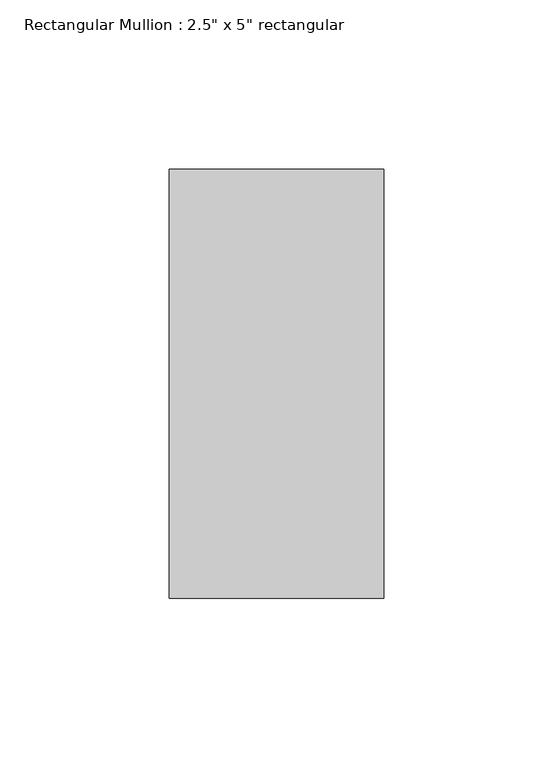
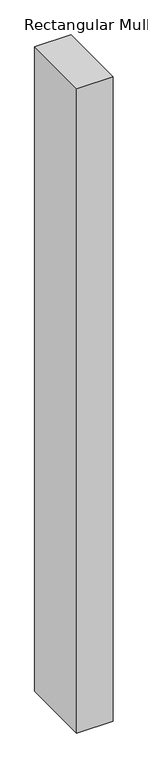
"""IFC4 building model written with IfcOpenShell, lengths in millimetres: member geometry."""

from ifc_helpers import new_model, si_unit, frame, origin, place, context, project, spatial, polyline, outline, extrude, source, transform, mapped, element, save


def member_c617b399(model_context):
    return source(origin(), model_context, "Body", "SweptSolid", [
        extrude(outline(polyline([(0.0, 63.5), (0.0, -63.5), (-63.5, -63.5), (-63.5, 63.5), (0.0, 63.5)])), frame((0.0, 0.0, -1188.8151287), z_axis=(0.0, 0.0, 1.0), x_axis=(1.0, 0.0, 0.0)), (0.0, 0.0, 1.0), 1188.8151287),
    ])


if __name__ == "__main__":
    model = new_model("IFC4")
    model_context = context("Model", 3, world=origin())
    ifc_project = project(units=[si_unit("LENGTHUNIT", "METRE", prefix="MILLI")], contexts=[model_context])
    site = spatial("IfcSite", under=ifc_project)
    building = spatial("IfcBuilding", under=site)
    placement = place(None, origin())
    member_shape = member_c617b399(model_context)
    element("IfcMember", 1, ObjectType="Rectangular Mullion : 2.5\" x 5\" rectangular", at=placement, inside=building, context=model_context, shape_type="MappedRepresentation", body=[
        mapped(member_shape, transform((0.0, 0.0, 0.0), x_axis=(1.0, 0.0, 0.0), y_axis=(0.0, 1.0, 0.0), z_axis=(0.0, 0.0, 1.0))),
    ])
    save(model, "model.ifc")

# Revit data of these elements
# Type "Rectangular Mullion : 2.5\" x 5\" rectangular"
#   built-in parameter 1007304 = 0.416667 (stored number, unit not read)
#   built-in parameter 1007301 = 0.104167 (stored number, unit not read)
#   built-in parameter 1007300 = 0.104167 (stored number, unit not read)
# Element 1 (IfcMember, "Rectangular Mullion : 2.5\" x 5\" rectangular")
#   Materials on its faces: "Metal - Aluminum"
# Materials
#   "Metal - Aluminum": class "Metal", colour RGB 140 140 140, transparency 0
